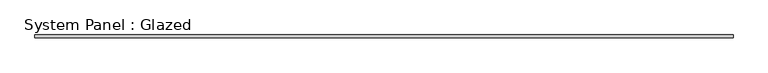
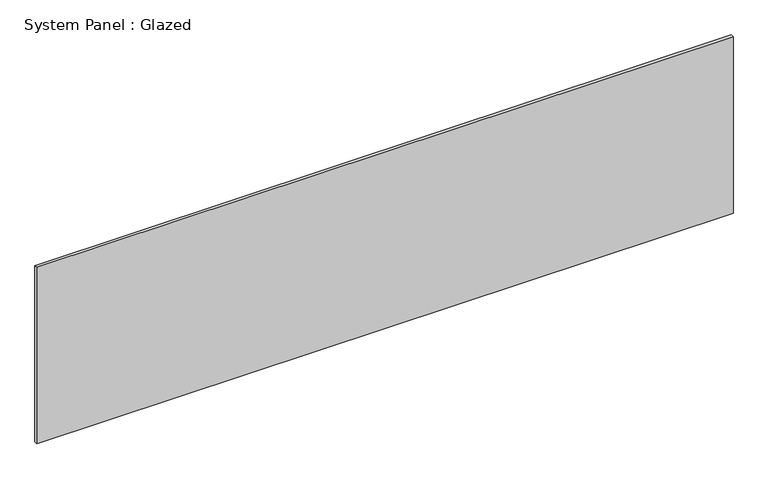
"""IFC4 building model written with IfcOpenShell, lengths in millimetres: plate geometry, System Panel : Glazed."""

import ifcopenshell
import ifcopenshell.guid

model = None  # the IFC model being written
_history = None  # IfcOwnerHistory: only IFC2X3 demands one
_inside = {}  # id of a spatial element -> (the spatial element, [elements in it])
_under = {}  # id of a project, library or spatial element -> (it, [spatial elements below it])
_declared = {}  # id of a project -> (the project, [libraries it declares])
_typed = {}  # id of a type object -> (the type object, [elements of that type])
_made_of = {}  # id of a material, layer set ... -> (it, [elements and type objects made of it])


def new_model(schema):
    """Start an empty IFC model of exactly this schema.

    Asked for "IFC4X3", IfcOpenShell would pick the latest addendum, in which some entities
    have other attributes; the version numbers below select the first issue.
    IFC2X3 requires an IfcOwnerHistory on every rooted entity: one is made here for all.
    """
    global model, _history
    if schema == "IFC4X3":
        model = ifcopenshell.file(schema_version=(4, 3, 0, 0))
    else:
        model = ifcopenshell.file(schema=schema)
    _inside.clear()
    _under.clear()
    _declared.clear()
    _typed.clear()
    _made_of.clear()
    _history = None
    if model.schema == "IFC2X3":
        org = make("IfcOrganization", Name="unknown")
        user = make(
            "IfcPersonAndOrganization",
            ThePerson=make("IfcPerson", FamilyName="unknown"),
            TheOrganization=org,
        )
        app = make(
            "IfcApplication",
            ApplicationDeveloper=org,
            Version="unknown",
            ApplicationFullName="unknown",
            ApplicationIdentifier="unknown",
        )
        _history = make(
            "IfcOwnerHistory",
            OwningUser=user,
            OwningApplication=app,
            ChangeAction="ADDED",
            CreationDate=0,
        )
    return model


def make(cls, **values):
    """One entity of the class cls with the attributes given. An attribute that is None is left unset."""
    return model.create_entity(
        cls, **{name: value for name, value in values.items() if value is not None}
    )


def rooted(cls, **values):
    """An entity with a GlobalId (a new one), such as an element, a storey or a relation."""
    return make(cls, GlobalId=ifcopenshell.guid.new(), OwnerHistory=_history, **values)


def si_unit(unit_type, name, prefix=None):
    """IfcSIUnit, for example si_unit("LENGTHUNIT", "METRE", prefix="MILLI")."""
    return make("IfcSIUnit", UnitType=unit_type, Prefix=prefix, Name=name)


def assignment(units):
    """IfcUnitAssignment: the units of a project."""
    return None if units is None else make("IfcUnitAssignment", Units=units)


def point(xyz):
    """IfcCartesianPoint."""
    return None if xyz is None else make("IfcCartesianPoint", Coordinates=xyz)


def direction(xyz):
    """IfcDirection."""
    return None if xyz is None else make("IfcDirection", DirectionRatios=xyz)


def frame(location, z_axis=None, x_axis=None):
    """IfcAxis2Placement3D, a coordinate frame: its origin and axes. An axis left out is left unset."""
    return make(
        "IfcAxis2Placement3D",
        Location=point(location),
        Axis=direction(z_axis),
        RefDirection=direction(x_axis),
    )


def origin():
    """The frame at (0, 0, 0) with its axes left unset."""
    return frame((0.0, 0.0, 0.0))


def origin_with_axes():
    """The frame at (0, 0, 0) with the z axis (0, 0, 1) and the x axis (1, 0, 0) written out."""
    return frame((0.0, 0.0, 0.0), z_axis=(0.0, 0.0, 1.0), x_axis=(1.0, 0.0, 0.0))


def place(relative_to, where):
    """IfcLocalPlacement: puts the frame where relative to a parent placement (None: the world)."""
    return make(
        "IfcLocalPlacement", PlacementRelTo=relative_to, RelativePlacement=where
    )


def context(
    kind, dimensions, precision=None, world=None, true_north=None, identifier=None
):
    """IfcGeometricRepresentationContext, for example the 3D "Model" context."""
    return make(
        "IfcGeometricRepresentationContext",
        ContextIdentifier=identifier,
        ContextType=kind,
        CoordinateSpaceDimension=dimensions,
        Precision=precision,
        WorldCoordinateSystem=world,
        TrueNorth=true_north,
    )


def project(units=None, contexts=None):
    """IfcProject with its units and contexts."""
    return rooted(
        "IfcProject",
        Name="project",
        RepresentationContexts=contexts,
        UnitsInContext=assignment(units),
    )


def spatial(cls, under=None, at=None, **own):
    """A site, building, storey or space (cls), placed at a placement, below another one or the project."""
    s = rooted(cls, ObjectPlacement=at, **own)
    if under is not None:
        _under.setdefault(under.id(), (under, []))[1].append(s)
    return s


def polyline(points):
    """IfcPolyline through the points."""
    return make("IfcPolyline", Points=[point(p) for p in points])


def outline(outer, holes=None, kind="AREA"):
    """IfcArbitraryClosedProfileDef: a profile drawn as a closed curve; with holes, ...WithVoids."""
    if holes is None:
        return make("IfcArbitraryClosedProfileDef", ProfileType=kind, OuterCurve=outer)
    return make(
        "IfcArbitraryProfileDefWithVoids",
        ProfileType=kind,
        OuterCurve=outer,
        InnerCurves=holes,
    )


def extrude(swept, where, along, depth):
    """IfcExtrudedAreaSolid: the profile swept, set in the frame where, extruded along a direction by depth."""
    return make(
        "IfcExtrudedAreaSolid",
        SweptArea=swept,
        Position=where,
        ExtrudedDirection=direction(along),
        Depth=depth,
    )


def shape(context_of_items, identifier, shape_type, items):
    """IfcShapeRepresentation: the items that make up one representation, for example the "Body"."""
    return make(
        "IfcShapeRepresentation",
        ContextOfItems=context_of_items,
        RepresentationIdentifier=identifier,
        RepresentationType=shape_type,
        Items=items,
    )


def source(mapping_origin, context_of_items, identifier, shape_type, items):
    """IfcRepresentationMap: a shape defined once, which mapped items show again and again."""
    return make(
        "IfcRepresentationMap",
        MappingOrigin=mapping_origin,
        MappedRepresentation=shape(context_of_items, identifier, shape_type, items),
    )


def transform(
    local_origin,
    x_axis=None,
    y_axis=None,
    z_axis=None,
    scale=None,
    scale2=None,
    scale3=None,
    uniform=True,
):
    """IfcCartesianTransformationOperator3D, or its non-uniform kind. x_axis, y_axis, z_axis: its Axis1, 2, 3."""
    if uniform:
        return make(
            "IfcCartesianTransformationOperator3D",
            Axis1=direction(x_axis),
            Axis2=direction(y_axis),
            LocalOrigin=point(local_origin),
            Scale=scale,
            Axis3=direction(z_axis),
        )
    return make(
        "IfcCartesianTransformationOperator3DnonUniform",
        Axis1=direction(x_axis),
        Axis2=direction(y_axis),
        LocalOrigin=point(local_origin),
        Scale=scale,
        Axis3=direction(z_axis),
        Scale2=scale2,
        Scale3=scale3,
    )


def mapped(mapping_source, mapping_target):
    """IfcMappedItem: shows the shape of a source again, moved by a transform."""
    return make(
        "IfcMappedItem", MappingSource=mapping_source, MappingTarget=mapping_target
    )


def made_of(thing, what):
    """Note that an element or type object is made of a material, layer set ...; save() writes the relation."""
    if what is not None:
        _made_of.setdefault(what.id(), (what, []))[1].append(thing)
    return thing


def element(
    cls,
    number,
    at=None,
    inside=None,
    cuts=None,
    type_object=None,
    material=None,
    context=None,
    identifier="Body",
    shape_type=None,
    held_by="IfcProductDefinitionShape",
    body=None,
    shapes=None,
    **own,
):
    """One element of the class cls, such as IfcWall. Its Tag is "e" and its number.

    at: its placement. inside: the storey or other place that contains it. cuts: it is an
    opening in that element (IfcRelVoidsElement). A single representation is given by context,
    identifier, shape_type and body (its items); several are given by shapes. held_by: the class
    of the entity that holds the representations. save() writes the other relations.
    """
    e = rooted(cls, Tag="e%d" % number, ObjectPlacement=at, **own)
    if body is not None:
        shapes = [shape(context, identifier, shape_type, body)]
    if shapes is not None:
        e.Representation = make(held_by, Representations=shapes)
    if inside is not None:
        _inside.setdefault(inside.id(), (inside, []))[1].append(e)
    if cuts is not None:
        rooted(
            "IfcRelVoidsElement", RelatingBuildingElement=cuts, RelatedOpeningElement=e
        )
    if type_object is not None:
        _typed.setdefault(type_object.id(), (type_object, []))[1].append(e)
    return made_of(e, material)


def aggregate(whole, parts):
    """IfcRelAggregates: a whole, such as a stair, and the parts it consists of."""
    return rooted("IfcRelAggregates", RelatingObject=whole, RelatedObjects=parts)


def save(model, path):
    """Write the relations noted so far, then the file.

    IfcRelAggregates (storeys below a building ...), IfcRelContainedInSpatialStructure (elements
    in a storey), IfcRelDefinesByType, IfcRelAssociatesMaterial and IfcRelDeclares: one each for
    every whole, place, type object, material and project.
    """
    for whole, parts in _under.values():
        aggregate(whole, parts)
    for where, things in _inside.values():
        rooted(
            "IfcRelContainedInSpatialStructure",
            RelatedElements=things,
            RelatingStructure=where,
        )
    for kind, things in _typed.values():
        rooted("IfcRelDefinesByType", RelatedObjects=things, RelatingType=kind)
    for what, things in _made_of.values():
        rooted("IfcRelAssociatesMaterial", RelatedObjects=things, RelatingMaterial=what)
    for by, libraries in _declared.values():
        rooted("IfcRelDeclares", RelatingContext=by, RelatedDefinitions=libraries)
    model.write(path)


def system_panel_glazed_40b49bdc(model_context):
    return source(origin(), model_context, "Body", "SweptSolid", [
        extrude(outline(polyline([(2850.0, 24.5), (-2850.0, 24.5), (-2850.0, 49.5), (2850.0, 49.5), (2850.0, 24.5)])), origin_with_axes(), (0.0, 0.0, 1.0), 1526.020449),
    ])


if __name__ == "__main__":
    model = new_model("IFC4")
    model_context = context("Model", 3, world=origin())
    ifc_project = project(units=[si_unit("LENGTHUNIT", "METRE", prefix="MILLI")], contexts=[model_context])
    site = spatial("IfcSite", under=ifc_project)
    building = spatial("IfcBuilding", under=site)
    placement = place(None, origin())
    system_panel_glazed_shape = system_panel_glazed_40b49bdc(model_context)
    element("IfcPlate", 1, ObjectType="System Panel : Glazed", at=placement, inside=building, context=model_context, shape_type="MappedRepresentation", body=[
        mapped(system_panel_glazed_shape, transform((0.0, 0.0, 0.0), x_axis=(1.0, 0.0, 0.0), y_axis=(0.0, 1.0, 0.0), z_axis=(0.0, 0.0, 1.0))),
    ])
    save(model, "model.ifc")

# Revit data of these elements
# Type "System Panel : Glazed"
#   Keynote = "H11"
#   Construction Type Id = "GSP4R"
#   Analytic Construction = "1/8 in Pilkington single glazing"
#   Visual Light Transmittance = 0.9
#   Solar Heat Gain Coefficient = 0.86
#   Heat Transfer Coefficient (U) = 6.7069 W/(m²·K)
#   Define Thermal Properties by = 1
# Element 1 (IfcPlate, "System Panel : Glazed")
#   Materials on its faces: "Glass"
# Materials
#   "Glass": class "Glass", colour RGB 0 128 192, transparency 0.9, Description = "Soda Lime Glass", Cost = 0
